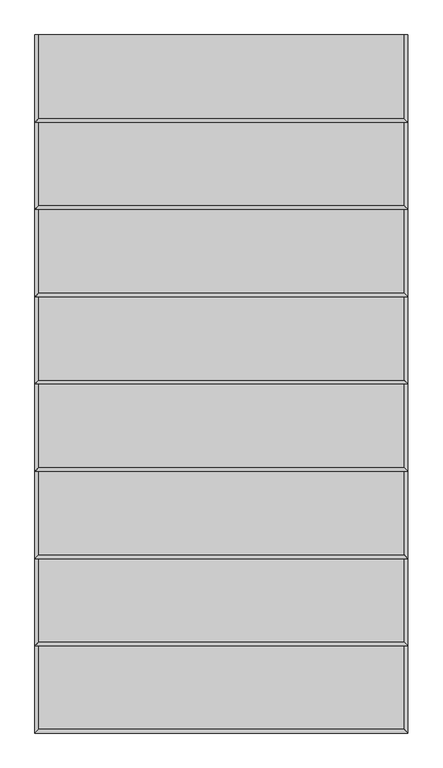
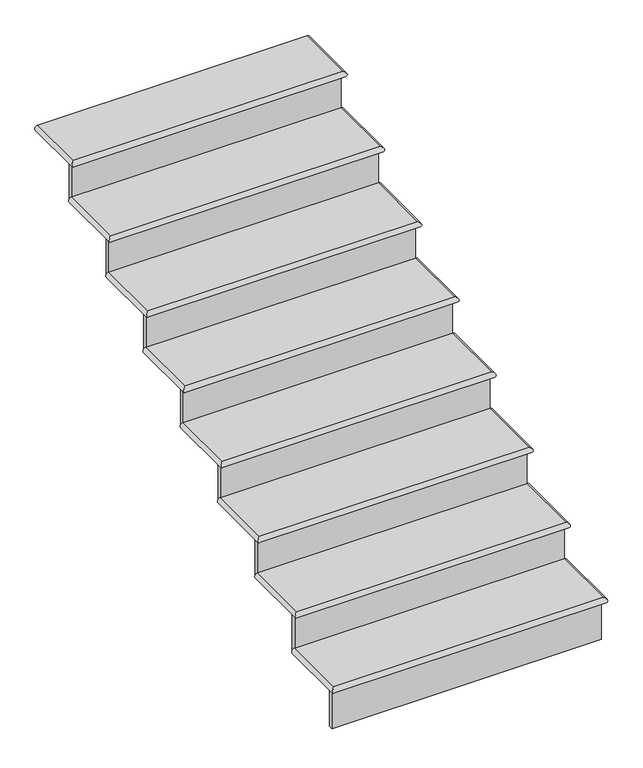
"""IFC4 building model written with IfcOpenShell, lengths in millimetres: stair flight geometry."""

from ifc_helpers import new_model, si_unit, frame, origin, place, context, project, spatial, circle_curve, ellipse_curve, faceted_brep, source, transform, mapped, element, save
from ifc_brep_helpers import plane_surface, cylinder_surface, advanced_brep


def stair_flight_4eb45a64(model_context):
    return source(origin(), model_context, "Body", "SolidModel", [
        advanced_brep(
        [(27169.2620052, 3880.9043237, 1549.796875), (27169.2620052, 3880.9043237, 1575.196875), (26000.8620052, 3880.9043237, 1575.196875), (26000.8620052, 3880.9043237, 1549.796875), (27169.2620052, 4173.0043237, 1575.196875), (26000.8620052, 4173.0043237, 1575.196875), (26000.8620052, 4173.0043237, 1549.796875), (27169.2620052, 4173.0043237, 1549.796875)],
        [
            (0, 1, ellipse_curve(frame((27169.2620052, 3880.9043237, 1562.496875), z_axis=(-0.7071067811865502, -0.7071067811865448, 0.0), x_axis=(0.7071067811865448, -0.7071067811865502, 0.0)), 17.9605122, 12.7)),
            (1, 2),
            (2, 3, ellipse_curve(frame((26000.8620052, 3880.9043237, 1562.496875), z_axis=(0.7071067811865448, -0.7071067811865502, 0.0), x_axis=(0.7071067811865501, 0.7071067811865448, 0.0)), 17.9605122, 12.7)),
            (3, 0),
            (4, 5),
            (5, 2),
            (1, 4),
            (6, 7),
            (7, 0),
            (3, 6),
            (4, 7, circle_curve(frame((27169.2620052, 4173.0043237, 1562.496875), z_axis=(0.0, 1.0, 0.0), x_axis=(-1.0, 0.0, 0.0)), 12.7)),
            (6, 5, circle_curve(frame((26000.8620052, 4173.0043237, 1562.496875), z_axis=(0.0, 1.0, 0.0), x_axis=(1.0, 0.0, 0.0)), 12.7)),
        ],
        [
            cylinder_surface(frame((27169.2620052, 3880.9043237, 1562.496875), z_axis=(1.0, 0.0, 0.0), x_axis=(0.0, 1.0, 0.0)), 12.7),
            plane_surface(frame((26000.8620052, 3868.2043237, 1575.196875), z_axis=(0.0, 0.0, 1.0), x_axis=(0.0, -1.0, 0.0))),
            plane_surface(frame((26000.8620052, 3868.2043237, 1549.796875), z_axis=(0.0, 0.0, -1.0), x_axis=(0.0, 1.0, 0.0))),
            plane_surface(frame((27169.2620052, 4173.0043237, 1575.196875), z_axis=(0.0, 1.0, 0.0), x_axis=(0.0, 0.0, -1.0))),
            cylinder_surface(frame((27169.2620052, 4173.0043237, 1562.496875), z_axis=(0.0, 1.0, 0.0), x_axis=(-1.0, 0.0, 0.0)), 12.7),
            cylinder_surface(frame((26000.8620052, 3880.9043237, 1562.496875), z_axis=(0.0, -1.0, 0.0), x_axis=(1.0, 0.0, 0.0)), 12.7),
        ],
        [
            (0, [[1, 2, 3, 4]]),
            (1, [[5, 6, -2, 7]]),
            (2, [[8, 9, -4, 10]]),
            (3, [[-5, 11, -8, 12]]),
            (4, [[-11, -7, -1, -9]]),
            (5, [[-3, -6, -12, -10]]),
        ],
    ),
        faceted_brep([(27169.2620052, 3893.6043237, 1549.796875), (27169.2620052, 3893.6043237, 1374.775), (27169.2620052, 3912.6543237, 1374.775), (27169.2620052, 3912.6543237, 1549.796875), (26000.8620052, 3893.6043237, 1549.796875), (26000.8620052, 3912.6543237, 1549.796875), (26000.8620052, 3912.6543237, 1374.775), (26000.8620052, 3893.6043237, 1374.775)], [[[0, 1, 2, 3]], [[4, 5, 6, 7]], [[1, 0, 4, 7]], [[2, 1, 7, 6]], [[3, 2, 6, 5]], [[0, 3, 5, 4]]]),
        faceted_brep([(27169.2620052, 4173.0043237, 1724.81875), (27169.2620052, 4173.0043237, 1549.796875), (27169.2620052, 4192.0543237, 1549.796875), (27169.2620052, 4192.0543237, 1724.81875), (26000.8620052, 4173.0043237, 1724.81875), (26000.8620052, 4192.0543237, 1724.81875), (26000.8620052, 4192.0543237, 1549.796875), (26000.8620052, 4173.0043237, 1549.796875)], [[[0, 1, 2, 3]], [[4, 5, 6, 7]], [[1, 0, 4, 7]], [[2, 1, 7, 6]], [[3, 2, 6, 5]], [[0, 3, 5, 4]]]),
        advanced_brep(
        [(27169.2620052, 4452.4043237, 1750.21875), (26000.8620052, 4452.4043237, 1750.21875), (26000.8620052, 4160.3043237, 1750.21875), (27169.2620052, 4160.3043237, 1750.21875), (26000.8620052, 4452.4043237, 1724.81875), (27169.2620052, 4452.4043237, 1724.81875), (27169.2620052, 4160.3043237, 1724.81875), (26000.8620052, 4160.3043237, 1724.81875)],
        [
            (0, 1),
            (1, 2),
            (2, 3),
            (3, 0),
            (4, 5),
            (5, 6),
            (6, 7),
            (7, 4),
            (0, 5, circle_curve(frame((27169.2620052, 4452.4043237, 1737.51875), z_axis=(0.0, 1.0, 0.0), x_axis=(-1.0, 0.0, 0.0)), 12.7)),
            (4, 1, circle_curve(frame((26000.8620052, 4452.4043237, 1737.51875), z_axis=(0.0, 1.0, 0.0), x_axis=(1.0, 0.0, 0.0)), 12.7)),
            (6, 3, ellipse_curve(frame((27169.2620052, 4160.3043237, 1737.51875), z_axis=(-0.7071067811865557, -0.7071067811865392, 0.0), x_axis=(0.7071067811865395, -0.7071067811865557, 0.0)), 17.9605122, 12.7)),
            (2, 7, ellipse_curve(frame((26000.8620052, 4160.3043237, 1737.51875), z_axis=(0.7071067811865392, -0.7071067811865558, 0.0), x_axis=(0.7071067811865558, 0.7071067811865391, 0.0)), 17.9605122, 12.7)),
        ],
        [
            plane_surface(frame((26000.8620052, 3868.2043237, 1750.21875), z_axis=(0.0, 0.0, 1.0), x_axis=(0.0, -1.0, 0.0))),
            plane_surface(frame((26000.8620052, 3868.2043237, 1724.81875), z_axis=(0.0, 0.0, -1.0), x_axis=(0.0, 1.0, 0.0))),
            plane_surface(frame((27169.2620052, 4452.4043237, 1750.21875), z_axis=(0.0, 1.0, 0.0), x_axis=(0.0, 0.0, -1.0))),
            cylinder_surface(frame((27169.2620052, 4160.3043237, 1737.51875), z_axis=(1.0, 0.0, 0.0), x_axis=(0.0, 1.0, 0.0)), 12.7),
            cylinder_surface(frame((27169.2620052, 4452.4043237, 1737.51875), z_axis=(0.0, 1.0, 0.0), x_axis=(-1.0, 0.0, 0.0)), 12.7),
            cylinder_surface(frame((26000.8620052, 4160.3043237, 1737.51875), z_axis=(0.0, -1.0, 0.0), x_axis=(1.0, 0.0, 0.0)), 12.7),
        ],
        [
            (0, [[1, 2, 3, 4]]),
            (1, [[5, 6, 7, 8]]),
            (2, [[-1, 9, -5, 10]]),
            (3, [[11, -3, 12, -7]]),
            (4, [[-9, -4, -11, -6]]),
            (5, [[-12, -2, -10, -8]]),
        ],
    ),
        faceted_brep([(27169.2620052, 4452.4043237, 1899.840625), (27169.2620052, 4452.4043237, 1724.81875), (27169.2620052, 4471.4543237, 1724.81875), (27169.2620052, 4471.4543237, 1899.840625), (26000.8620052, 4452.4043237, 1899.840625), (26000.8620052, 4471.4543237, 1899.840625), (26000.8620052, 4471.4543237, 1724.81875), (26000.8620052, 4452.4043237, 1724.81875)], [[[0, 1, 2, 3]], [[4, 5, 6, 7]], [[1, 0, 4, 7]], [[2, 1, 7, 6]], [[3, 2, 6, 5]], [[0, 3, 5, 4]]]),
        advanced_brep(
        [(27169.2620052, 4731.8043237, 1925.240625), (26000.8620052, 4731.8043237, 1925.240625), (26000.8620052, 4439.7043237, 1925.240625), (27169.2620052, 4439.7043237, 1925.240625), (26000.8620052, 4731.8043237, 1899.840625), (27169.2620052, 4731.8043237, 1899.840625), (27169.2620052, 4439.7043237, 1899.840625), (26000.8620052, 4439.7043237, 1899.840625)],
        [
            (0, 1),
            (1, 2),
            (2, 3),
            (3, 0),
            (4, 5),
            (5, 6),
            (6, 7),
            (7, 4),
            (0, 5, circle_curve(frame((27169.2620052, 4731.8043237, 1912.540625), z_axis=(0.0, 1.0, 0.0), x_axis=(-1.0, 0.0, 0.0)), 12.7)),
            (4, 1, circle_curve(frame((26000.8620052, 4731.8043237, 1912.540625), z_axis=(0.0, 1.0, 0.0), x_axis=(1.0, 0.0, 0.0)), 12.7)),
            (6, 3, ellipse_curve(frame((27169.2620052, 4439.7043237, 1912.540625), z_axis=(-0.7071067811865557, -0.7071067811865392, 0.0), x_axis=(0.7071067811865395, -0.7071067811865557, 0.0)), 17.9605122, 12.7)),
            (2, 7, ellipse_curve(frame((26000.8620052, 4439.7043237, 1912.540625), z_axis=(0.7071067811865392, -0.7071067811865558, 0.0), x_axis=(0.7071067811865558, 0.7071067811865391, 0.0)), 17.9605122, 12.7)),
        ],
        [
            plane_surface(frame((26000.8620052, 4147.6043237, 1925.240625), z_axis=(0.0, 0.0, 1.0), x_axis=(0.0, -1.0, 0.0))),
            plane_surface(frame((26000.8620052, 4147.6043237, 1899.840625), z_axis=(0.0, 0.0, -1.0), x_axis=(0.0, 1.0, 0.0))),
            plane_surface(frame((27169.2620052, 4731.8043237, 1925.240625), z_axis=(0.0, 1.0, 0.0), x_axis=(0.0, 0.0, -1.0))),
            cylinder_surface(frame((27169.2620052, 4439.7043237, 1912.540625), z_axis=(1.0, 0.0, 0.0), x_axis=(0.0, 1.0, 0.0)), 12.7),
            cylinder_surface(frame((27169.2620052, 4731.8043237, 1912.540625), z_axis=(0.0, 1.0, 0.0), x_axis=(-1.0, 0.0, 0.0)), 12.7),
            cylinder_surface(frame((26000.8620052, 4439.7043237, 1912.540625), z_axis=(0.0, -1.0, 0.0), x_axis=(1.0, 0.0, 0.0)), 12.7),
        ],
        [
            (0, [[1, 2, 3, 4]]),
            (1, [[5, 6, 7, 8]]),
            (2, [[-1, 9, -5, 10]]),
            (3, [[11, -3, 12, -7]]),
            (4, [[-9, -4, -11, -6]]),
            (5, [[-12, -2, -10, -8]]),
        ],
    ),
        faceted_brep([(27169.2620052, 4731.8043237, 2074.8625), (27169.2620052, 4731.8043237, 1899.840625), (27169.2620052, 4750.8543237, 1899.840625), (27169.2620052, 4750.8543237, 2074.8625), (26000.8620052, 4731.8043237, 2074.8625), (26000.8620052, 4750.8543237, 2074.8625), (26000.8620052, 4750.8543237, 1899.840625), (26000.8620052, 4731.8043237, 1899.840625)], [[[0, 1, 2, 3]], [[4, 5, 6, 7]], [[1, 0, 4, 7]], [[2, 1, 7, 6]], [[3, 2, 6, 5]], [[0, 3, 5, 4]]]),
        advanced_brep(
        [(27169.2620052, 5011.2043237, 2100.2625), (26000.8620052, 5011.2043237, 2100.2625), (26000.8620052, 4719.1043237, 2100.2625), (27169.2620052, 4719.1043237, 2100.2625), (26000.8620052, 5011.2043237, 2074.8625), (27169.2620052, 5011.2043237, 2074.8625), (27169.2620052, 4719.1043237, 2074.8625), (26000.8620052, 4719.1043237, 2074.8625)],
        [
            (0, 1),
            (1, 2),
            (2, 3),
            (3, 0),
            (4, 5),
            (5, 6),
            (6, 7),
            (7, 4),
            (0, 5, circle_curve(frame((27169.2620052, 5011.2043237, 2087.5625), z_axis=(0.0, 1.0, 0.0), x_axis=(-1.0, 0.0, 0.0)), 12.7)),
            (4, 1, circle_curve(frame((26000.8620052, 5011.2043237, 2087.5625), z_axis=(0.0, 1.0, 0.0), x_axis=(1.0, 0.0, 0.0)), 12.7)),
            (6, 3, ellipse_curve(frame((27169.2620052, 4719.1043237, 2087.5625), z_axis=(-0.7071067811865557, -0.7071067811865392, 0.0), x_axis=(0.7071067811865395, -0.7071067811865557, 0.0)), 17.9605122, 12.7)),
            (2, 7, ellipse_curve(frame((26000.8620052, 4719.1043237, 2087.5625), z_axis=(0.7071067811865392, -0.7071067811865558, 0.0), x_axis=(0.7071067811865558, 0.7071067811865391, 0.0)), 17.9605122, 12.7)),
        ],
        [
            plane_surface(frame((26000.8620052, 4427.0043237, 2100.2625), z_axis=(0.0, 0.0, 1.0), x_axis=(0.0, -1.0, 0.0))),
            plane_surface(frame((26000.8620052, 4427.0043237, 2074.8625), z_axis=(0.0, 0.0, -1.0), x_axis=(0.0, 1.0, 0.0))),
            plane_surface(frame((27169.2620052, 5011.2043237, 2100.2625), z_axis=(0.0, 1.0, 0.0), x_axis=(0.0, 0.0, -1.0))),
            cylinder_surface(frame((27169.2620052, 4719.1043237, 2087.5625), z_axis=(1.0, 0.0, 0.0), x_axis=(0.0, 1.0, 0.0)), 12.7),
            cylinder_surface(frame((27169.2620052, 5011.2043237, 2087.5625), z_axis=(0.0, 1.0, 0.0), x_axis=(-1.0, 0.0, 0.0)), 12.7),
            cylinder_surface(frame((26000.8620052, 4719.1043237, 2087.5625), z_axis=(0.0, -1.0, 0.0), x_axis=(1.0, 0.0, 0.0)), 12.7),
        ],
        [
            (0, [[1, 2, 3, 4]]),
            (1, [[5, 6, 7, 8]]),
            (2, [[-1, 9, -5, 10]]),
            (3, [[11, -3, 12, -7]]),
            (4, [[-9, -4, -11, -6]]),
            (5, [[-12, -2, -10, -8]]),
        ],
    ),
        faceted_brep([(27169.2620052, 5011.2043237, 2249.884375), (27169.2620052, 5011.2043237, 2074.8625), (27169.2620052, 5030.2543237, 2074.8625), (27169.2620052, 5030.2543237, 2249.884375), (26000.8620052, 5011.2043237, 2249.884375), (26000.8620052, 5030.2543237, 2249.884375), (26000.8620052, 5030.2543237, 2074.8625), (26000.8620052, 5011.2043237, 2074.8625)], [[[0, 1, 2, 3]], [[4, 5, 6, 7]], [[1, 0, 4, 7]], [[2, 1, 7, 6]], [[3, 2, 6, 5]], [[0, 3, 5, 4]]]),
        advanced_brep(
        [(27169.2620052, 5290.6043237, 2275.284375), (26000.8620052, 5290.6043237, 2275.284375), (26000.8620052, 4998.5043237, 2275.284375), (27169.2620052, 4998.5043237, 2275.284375), (26000.8620052, 5290.6043237, 2249.884375), (27169.2620052, 5290.6043237, 2249.884375), (27169.2620052, 4998.5043237, 2249.884375), (26000.8620052, 4998.5043237, 2249.884375)],
        [
            (0, 1),
            (1, 2),
            (2, 3),
            (3, 0),
            (4, 5),
            (5, 6),
            (6, 7),
            (7, 4),
            (0, 5, circle_curve(frame((27169.2620052, 5290.6043237, 2262.584375), z_axis=(0.0, 1.0, 0.0), x_axis=(-1.0, 0.0, 0.0)), 12.7)),
            (4, 1, circle_curve(frame((26000.8620052, 5290.6043237, 2262.584375), z_axis=(0.0, 1.0, 0.0), x_axis=(1.0, 0.0, 0.0)), 12.7)),
            (6, 3, ellipse_curve(frame((27169.2620052, 4998.5043237, 2262.584375), z_axis=(-0.7071067811865557, -0.7071067811865392, 0.0), x_axis=(0.7071067811865395, -0.7071067811865557, 0.0)), 17.9605122, 12.7)),
            (2, 7, ellipse_curve(frame((26000.8620052, 4998.5043237, 2262.584375), z_axis=(0.7071067811865392, -0.7071067811865558, 0.0), x_axis=(0.7071067811865558, 0.7071067811865391, 0.0)), 17.9605122, 12.7)),
        ],
        [
            plane_surface(frame((26000.8620052, 4706.4043237, 2275.284375), z_axis=(0.0, 0.0, 1.0), x_axis=(0.0, -1.0, 0.0))),
            plane_surface(frame((26000.8620052, 4706.4043237, 2249.884375), z_axis=(0.0, 0.0, -1.0), x_axis=(0.0, 1.0, 0.0))),
            plane_surface(frame((27169.2620052, 5290.6043237, 2275.284375), z_axis=(0.0, 1.0, 0.0), x_axis=(0.0, 0.0, -1.0))),
            cylinder_surface(frame((27169.2620052, 4998.5043237, 2262.584375), z_axis=(1.0, 0.0, 0.0), x_axis=(0.0, 1.0, 0.0)), 12.7),
            cylinder_surface(frame((27169.2620052, 5290.6043237, 2262.584375), z_axis=(0.0, 1.0, 0.0), x_axis=(-1.0, 0.0, 0.0)), 12.7),
            cylinder_surface(frame((26000.8620052, 4998.5043237, 2262.584375), z_axis=(0.0, -1.0, 0.0), x_axis=(1.0, 0.0, 0.0)), 12.7),
        ],
        [
            (0, [[1, 2, 3, 4]]),
            (1, [[5, 6, 7, 8]]),
            (2, [[-1, 9, -5, 10]]),
            (3, [[11, -3, 12, -7]]),
            (4, [[-9, -4, -11, -6]]),
            (5, [[-12, -2, -10, -8]]),
        ],
    ),
        faceted_brep([(27169.2620052, 5290.6043237, 2424.90625), (27169.2620052, 5290.6043237, 2249.884375), (27169.2620052, 5309.6543237, 2249.884375), (27169.2620052, 5309.6543237, 2424.90625), (26000.8620052, 5290.6043237, 2424.90625), (26000.8620052, 5309.6543237, 2424.90625), (26000.8620052, 5309.6543237, 2249.884375), (26000.8620052, 5290.6043237, 2249.884375)], [[[0, 1, 2, 3]], [[4, 5, 6, 7]], [[1, 0, 4, 7]], [[2, 1, 7, 6]], [[3, 2, 6, 5]], [[0, 3, 5, 4]]]),
        advanced_brep(
        [(27169.2620052, 5570.0043237, 2450.30625), (26000.8620052, 5570.0043237, 2450.30625), (26000.8620052, 5277.9043237, 2450.30625), (27169.2620052, 5277.9043237, 2450.30625), (26000.8620052, 5570.0043237, 2424.90625), (27169.2620052, 5570.0043237, 2424.90625), (27169.2620052, 5277.9043237, 2424.90625), (26000.8620052, 5277.9043237, 2424.90625)],
        [
            (0, 1),
            (1, 2),
            (2, 3),
            (3, 0),
            (4, 5),
            (5, 6),
            (6, 7),
            (7, 4),
            (0, 5, circle_curve(frame((27169.2620052, 5570.0043237, 2437.60625), z_axis=(0.0, 1.0, 0.0), x_axis=(-1.0, 0.0, 0.0)), 12.7)),
            (4, 1, circle_curve(frame((26000.8620052, 5570.0043237, 2437.60625), z_axis=(0.0, 1.0, 0.0), x_axis=(1.0, 0.0, 0.0)), 12.7)),
            (6, 3, ellipse_curve(frame((27169.2620052, 5277.9043237, 2437.60625), z_axis=(-0.7071067811865557, -0.7071067811865392, 0.0), x_axis=(0.7071067811865395, -0.7071067811865557, 0.0)), 17.9605122, 12.7)),
            (2, 7, ellipse_curve(frame((26000.8620052, 5277.9043237, 2437.60625), z_axis=(0.7071067811865392, -0.7071067811865558, 0.0), x_axis=(0.7071067811865558, 0.7071067811865391, 0.0)), 17.9605122, 12.7)),
        ],
        [
            plane_surface(frame((26000.8620052, 4985.8043237, 2450.30625), z_axis=(0.0, 0.0, 1.0), x_axis=(0.0, -1.0, 0.0))),
            plane_surface(frame((26000.8620052, 4985.8043237, 2424.90625), z_axis=(0.0, 0.0, -1.0), x_axis=(0.0, 1.0, 0.0))),
            plane_surface(frame((27169.2620052, 5570.0043237, 2450.30625), z_axis=(0.0, 1.0, 0.0), x_axis=(0.0, 0.0, -1.0))),
            cylinder_surface(frame((27169.2620052, 5277.9043237, 2437.60625), z_axis=(1.0, 0.0, 0.0), x_axis=(0.0, 1.0, 0.0)), 12.7),
            cylinder_surface(frame((27169.2620052, 5570.0043237, 2437.60625), z_axis=(0.0, 1.0, 0.0), x_axis=(-1.0, 0.0, 0.0)), 12.7),
            cylinder_surface(frame((26000.8620052, 5277.9043237, 2437.60625), z_axis=(0.0, -1.0, 0.0), x_axis=(1.0, 0.0, 0.0)), 12.7),
        ],
        [
            (0, [[1, 2, 3, 4]]),
            (1, [[5, 6, 7, 8]]),
            (2, [[-1, 9, -5, 10]]),
            (3, [[11, -3, 12, -7]]),
            (4, [[-9, -4, -11, -6]]),
            (5, [[-12, -2, -10, -8]]),
        ],
    ),
        faceted_brep([(27169.2620052, 5570.0043237, 2599.928125), (27169.2620052, 5570.0043237, 2424.90625), (27169.2620052, 5589.0543237, 2424.90625), (27169.2620052, 5589.0543237, 2599.928125), (26000.8620052, 5570.0043237, 2599.928125), (26000.8620052, 5589.0543237, 2599.928125), (26000.8620052, 5589.0543237, 2424.90625), (26000.8620052, 5570.0043237, 2424.90625)], [[[0, 1, 2, 3]], [[4, 5, 6, 7]], [[1, 0, 4, 7]], [[2, 1, 7, 6]], [[3, 2, 6, 5]], [[0, 3, 5, 4]]]),
        advanced_brep(
        [(27169.2620052, 5849.4043237, 2625.328125), (26000.8620052, 5849.4043237, 2625.328125), (26000.8620052, 5557.3043237, 2625.328125), (27169.2620052, 5557.3043237, 2625.328125), (26000.8620052, 5849.4043237, 2599.928125), (27169.2620052, 5849.4043237, 2599.928125), (27169.2620052, 5557.3043237, 2599.928125), (26000.8620052, 5557.3043237, 2599.928125)],
        [
            (0, 1),
            (1, 2),
            (2, 3),
            (3, 0),
            (4, 5),
            (5, 6),
            (6, 7),
            (7, 4),
            (0, 5, circle_curve(frame((27169.2620052, 5849.4043237, 2612.628125), z_axis=(0.0, 1.0, 0.0), x_axis=(-1.0, 0.0, 0.0)), 12.7)),
            (4, 1, circle_curve(frame((26000.8620052, 5849.4043237, 2612.628125), z_axis=(0.0, 1.0, 0.0), x_axis=(1.0, 0.0, 0.0)), 12.7)),
            (6, 3, ellipse_curve(frame((27169.2620052, 5557.3043237, 2612.628125), z_axis=(-0.7071067811865557, -0.7071067811865392, 0.0), x_axis=(0.7071067811865395, -0.7071067811865557, 0.0)), 17.9605122, 12.7)),
            (2, 7, ellipse_curve(frame((26000.8620052, 5557.3043237, 2612.628125), z_axis=(0.7071067811865392, -0.7071067811865558, 0.0), x_axis=(0.7071067811865558, 0.7071067811865391, 0.0)), 17.9605122, 12.7)),
        ],
        [
            plane_surface(frame((26000.8620052, 5265.2043237, 2625.328125), z_axis=(0.0, 0.0, 1.0), x_axis=(0.0, -1.0, 0.0))),
            plane_surface(frame((26000.8620052, 5265.2043237, 2599.928125), z_axis=(0.0, 0.0, -1.0), x_axis=(0.0, 1.0, 0.0))),
            plane_surface(frame((27169.2620052, 5849.4043237, 2625.328125), z_axis=(0.0, 1.0, 0.0), x_axis=(0.0, 0.0, -1.0))),
            cylinder_surface(frame((27169.2620052, 5557.3043237, 2612.628125), z_axis=(1.0, 0.0, 0.0), x_axis=(0.0, 1.0, 0.0)), 12.7),
            cylinder_surface(frame((27169.2620052, 5849.4043237, 2612.628125), z_axis=(0.0, 1.0, 0.0), x_axis=(-1.0, 0.0, 0.0)), 12.7),
            cylinder_surface(frame((26000.8620052, 5557.3043237, 2612.628125), z_axis=(0.0, -1.0, 0.0), x_axis=(1.0, 0.0, 0.0)), 12.7),
        ],
        [
            (0, [[1, 2, 3, 4]]),
            (1, [[5, 6, 7, 8]]),
            (2, [[-1, 9, -5, 10]]),
            (3, [[11, -3, 12, -7]]),
            (4, [[-9, -4, -11, -6]]),
            (5, [[-12, -2, -10, -8]]),
        ],
    ),
        faceted_brep([(27169.2620052, 5849.4043237, 2774.95), (27169.2620052, 5849.4043237, 2599.928125), (27169.2620052, 5868.4543237, 2599.928125), (27169.2620052, 5868.4543237, 2774.95), (26000.8620052, 5849.4043237, 2774.95), (26000.8620052, 5868.4543237, 2774.95), (26000.8620052, 5868.4543237, 2599.928125), (26000.8620052, 5849.4043237, 2599.928125)], [[[0, 1, 2, 3]], [[4, 5, 6, 7]], [[1, 0, 4, 7]], [[2, 1, 7, 6]], [[3, 2, 6, 5]], [[0, 3, 5, 4]]]),
        advanced_brep(
        [(27169.2620052, 6103.4043237, 2800.35), (26000.8620052, 6103.4043237, 2800.35), (26000.8620052, 5836.7043237, 2800.35), (27169.2620052, 5836.7043237, 2800.35), (26000.8620052, 6103.4043237, 2774.95), (27169.2620052, 6103.4043237, 2774.95), (27169.2620052, 5836.7043237, 2774.95), (26000.8620052, 5836.7043237, 2774.95)],
        [
            (0, 1),
            (1, 2),
            (2, 3),
            (3, 0),
            (4, 5),
            (5, 6),
            (6, 7),
            (7, 4),
            (0, 5, circle_curve(frame((27169.2620052, 6103.4043237, 2787.65), z_axis=(0.0, 1.0, 0.0), x_axis=(-1.0, 0.0, 0.0)), 12.7)),
            (4, 1, circle_curve(frame((26000.8620052, 6103.4043237, 2787.65), z_axis=(0.0, 1.0, 0.0), x_axis=(1.0, 0.0, 0.0)), 12.7)),
            (3, 6, ellipse_curve(frame((27169.2620052, 5836.7043237, 2787.65), z_axis=(0.7071067811865557, 0.7071067811865392, 0.0), x_axis=(-0.7071067811865391, 0.7071067811865559, 0.0)), 17.9605122, 12.7)),
            (2, 7, ellipse_curve(frame((26000.8620052, 5836.7043237, 2787.65), z_axis=(0.7071067811865392, -0.7071067811865558, 0.0), x_axis=(0.7071067811865558, 0.7071067811865391, 0.0)), 17.9605122, 12.7)),
        ],
        [
            plane_surface(frame((26000.8620052, 3868.2043237, 2800.35), z_axis=(0.0, 0.0, 1.0), x_axis=(0.0, -1.0, 0.0))),
            plane_surface(frame((26000.8620052, 3868.2043237, 2774.95), z_axis=(0.0, 0.0, -1.0), x_axis=(0.0, 1.0, 0.0))),
            plane_surface(frame((27169.2620052, 6103.4043237, 2800.35), z_axis=(0.0, 1.0, 0.0), x_axis=(0.0, 0.0, -1.0))),
            cylinder_surface(frame((27169.2620052, 6103.4043237, 2787.65), z_axis=(0.0, 1.0, 0.0), x_axis=(-1.0, 0.0, 0.0)), 12.7),
            cylinder_surface(frame((27169.2620052, 5836.7043237, 2787.65), z_axis=(1.0, 0.0, 0.0), x_axis=(0.0, 1.0, 0.0)), 12.7),
            cylinder_surface(frame((26000.8620052, 5836.7043237, 2787.65), z_axis=(0.0, -1.0, 0.0), x_axis=(1.0, 0.0, 0.0)), 12.7),
        ],
        [
            (0, [[1, 2, 3, 4]]),
            (1, [[5, 6, 7, 8]]),
            (2, [[-1, 9, -5, 10]]),
            (3, [[-9, -4, 11, -6]]),
            (4, [[-11, -3, 12, -7]]),
            (5, [[-12, -2, -10, -8]]),
        ],
    ),
    ])


if __name__ == "__main__":
    model = new_model("IFC4")
    model_context = context("Model", 3, world=origin())
    ifc_project = project(units=[si_unit("LENGTHUNIT", "METRE", prefix="MILLI")], contexts=[model_context])
    site = spatial("IfcSite", under=ifc_project)
    building = spatial("IfcBuilding", under=site)
    placement = place(None, origin())
    stair_flight_shape = stair_flight_4eb45a64(model_context)
    element("IfcStairFlight", 1, at=placement, inside=building, context=model_context, shape_type="MappedRepresentation", body=[
        mapped(stair_flight_shape, transform((0.0, 0.0, 0.0), x_axis=(1.0, 0.0, 0.0), y_axis=(0.0, 1.0, 0.0), z_axis=(0.0, 0.0, 1.0))),
    ])
    save(model, "model.ifc")

# Revit data of these elements
# Element 1 (IfcStairFlight)
#   Materials on its faces: "FINISH T.B.D."
# Materials
#   "FINISH T.B.D.": class "Generic", colour RGB 227 188 136, transparency 0, Cost = 0
